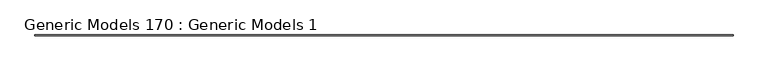
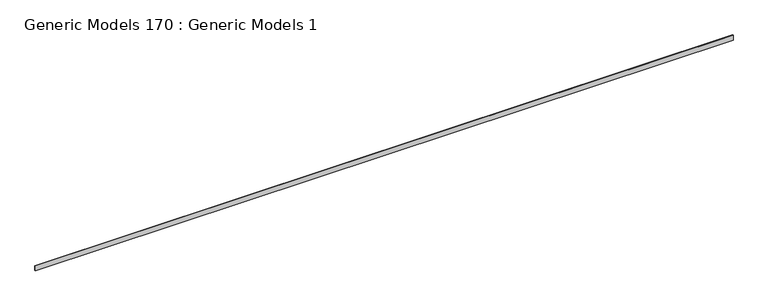
"""IFC4 building model written with IfcOpenShell, lengths in millimetres: proxy geometry, Generic Models 170 : Generic Models 1."""

from ifc_helpers import new_model, si_unit, frame, origin, place, context, project, spatial, polyline, outline, extrude, source, transform, mapped, element, save


def generic_models_170_generic_models_1_e453f141(model_context):
    return source(origin(), model_context, "Body", "SweptSolid", [
        extrude(outline(polyline([(-5273.7375551, 126783.846), (-5292.7875551, 126783.846), (-5292.7875551, 126923.546), (-5274.9281801, 126923.546), (-5273.7375551, 126922.355375), (-5273.7375551, 126783.846)])), frame((-16853.0736296, 0.0, 0.0), z_axis=(1.0, 0.0, 0.0), x_axis=(0.0, 1.0, 0.0)), (0.0, 0.0, 1.0), 19050.0),
    ])


if __name__ == "__main__":
    model = new_model("IFC4")
    model_context = context("Model", 3, world=origin())
    ifc_project = project(units=[si_unit("LENGTHUNIT", "METRE", prefix="MILLI")], contexts=[model_context])
    site = spatial("IfcSite", under=ifc_project)
    building = spatial("IfcBuilding", under=site)
    placement = place(None, origin())
    generic_models_170_generic_models_1_shape = generic_models_170_generic_models_1_e453f141(model_context)
    element("IfcBuildingElementProxy", 1, Name="Generic Models 170 : Generic Models 1", ObjectType="Generic Models 170 : Generic Models 1", at=placement, inside=building, context=model_context, shape_type="MappedRepresentation", body=[
        mapped(generic_models_170_generic_models_1_shape, transform((0.0, 0.0, 0.0), x_axis=(1.0, 0.0, 0.0), y_axis=(0.0, 1.0, 0.0), z_axis=(0.0, 0.0, 1.0))),
    ])
    save(model, "model.ifc")

# Revit data of these elements
# Element 1 (IfcBuildingElementProxy, "Generic Models 170 : Generic Models 1")
#   Materials on its faces: "_BASE TRIM AS SCHEDULED"
# Materials
#   "_BASE TRIM AS SCHEDULED": class "Generic", colour RGB 177 130 114, transparency 0, Cost = 0
